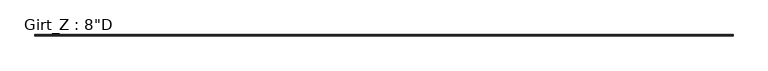
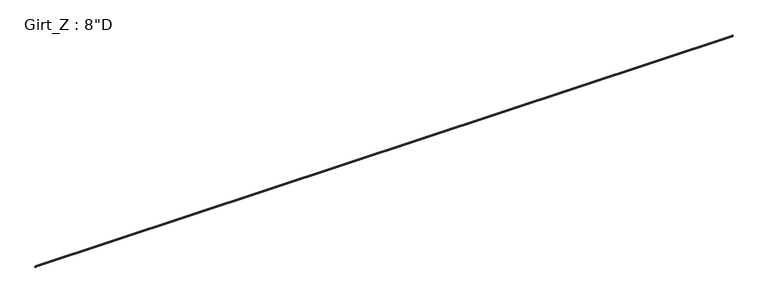
"""IFC4 building model written with IfcOpenShell, lengths in millimetres: beam geometry."""

from ifc_helpers import new_model, si_unit, point, frame, frame_2d, origin, place, context, project, spatial, polyline, circle_curve, trimmed, segment, composite_curve, outline, extrude, source, transform, mapped, element, save


def beam_e27b546e(model_context):
    return source(origin(), model_context, "Body", "SweptSolid", [
        extrude(outline(composite_curve([segment(polyline([(-63.5, 101.6), (-3.3734375, 101.6)]), True, "CONTINUOUS"), segment(trimmed(circle_curve(frame_2d((-3.3734375, 96.8375)), 4.7625), [point((-3.3734375, 101.6))], [point((1.3890625, 96.8375))], False, "CARTESIAN"), True, "CONTINUOUS"), segment(polyline([(1.3890625, 96.8375), (1.3890625, -96.8389339)]), True, "CONTINUOUS"), segment(trimmed(circle_curve(frame_2d((3.3748024, -96.8389339)), 1.9857399), [point((1.3890625, -96.8389339))], [point((3.2694106, -98.821875))], True, "CARTESIAN"), True, "CONTINUOUS"), segment(polyline([(3.2694106, -98.821875), (62.204539, -98.821875), (73.6169367, -85.221109), (75.745104, -87.0068534), (63.5, -101.6), (3.3734375, -101.6)]), True, "CONTINUOUS"), segment(trimmed(circle_curve(frame_2d((3.3734375, -96.8375)), 4.7625), [point((3.3734375, -101.6))], [point((-1.3890625, -96.8375))], False, "CARTESIAN"), True, "CONTINUOUS"), segment(polyline([(-1.3890625, -96.8375), (-1.3890625, 96.8381931)]), True, "CONTINUOUS"), segment(trimmed(circle_curve(frame_2d((-3.3741066, 96.8381931)), 1.9850441), [point((-1.3890625, 96.8381931))], [point((-3.3005807, 98.821875))], True, "CARTESIAN"), True, "CONTINUOUS"), segment(polyline([(-3.3005807, 98.821875), (-62.204539, 98.821875), (-73.6169367, 85.221109), (-75.745104, 87.0068534), (-63.5, 101.6)]), True, "CONTINUOUS")], self_intersect=False)), frame((-40669.2447266, 0.0, 0.0), z_axis=(1.0, 0.0, 0.0), x_axis=(0.0, 1.0, 0.0)), (0.0, 0.0, 1.0), 80870.1769531),
    ])


if __name__ == "__main__":
    model = new_model("IFC4")
    model_context = context("Model", 3, world=origin())
    ifc_project = project(units=[si_unit("LENGTHUNIT", "METRE", prefix="MILLI")], contexts=[model_context])
    site = spatial("IfcSite", under=ifc_project)
    building = spatial("IfcBuilding", under=site)
    placement = place(None, origin())
    beam_shape = beam_e27b546e(model_context)
    element("IfcBeam", 1, ObjectType="Girt_Z : 8\"D", at=placement, inside=building, context=model_context, shape_type="MappedRepresentation", body=[
        mapped(beam_shape, transform((0.0, 0.0, 0.0), x_axis=(1.0, 0.0, 0.0), y_axis=(0.0, 1.0, 0.0), z_axis=(0.0, 0.0, 1.0))),
    ])
    save(model, "model.ifc")

# Revit data of these elements
# Type "Girt_Z : 8\"D"
#   Web_Thickness = 0' - 0 7/64"
#   Length [instance default] = 10' - 0"
#   Leg_1 = 0' - 2 1/2"
#   Height = 0' - 8"
#   Structural Material [instance default] = none
# Element 1 (IfcBeam, "Girt_Z : 8\"D")
#   Structural Material = Steel
#   Materials on its faces: "Steel"
# Materials
#   "Steel": class "Metal", colour RGB 118 118 114, transparency 0, Description = "Steel, mill finish", Cost = 0
